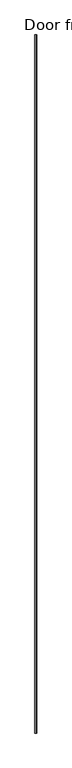
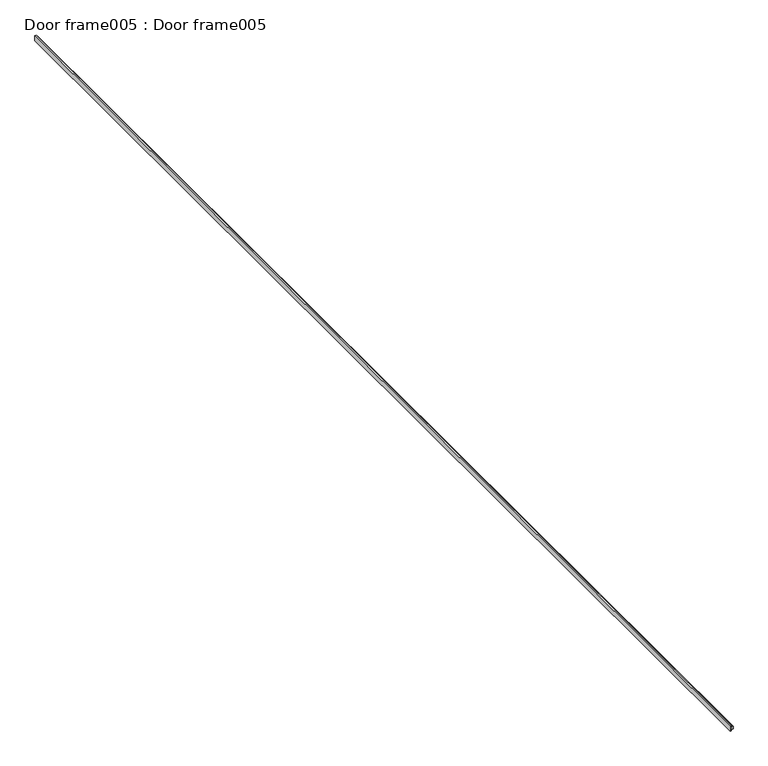
"""IFC4 building model written with IfcOpenShell, lengths in millimetres: proxy geometry, Door frame005 : Door frame005."""

import ifcopenshell
import ifcopenshell.guid

model = None  # the IFC model being written
_history = None  # IfcOwnerHistory: only IFC2X3 demands one
_inside = {}  # id of a spatial element -> (the spatial element, [elements in it])
_under = {}  # id of a project, library or spatial element -> (it, [spatial elements below it])
_declared = {}  # id of a project -> (the project, [libraries it declares])
_typed = {}  # id of a type object -> (the type object, [elements of that type])
_made_of = {}  # id of a material, layer set ... -> (it, [elements and type objects made of it])


def new_model(schema):
    """Start an empty IFC model of exactly this schema.

    Asked for "IFC4X3", IfcOpenShell would pick the latest addendum, in which some entities
    have other attributes; the version numbers below select the first issue.
    IFC2X3 requires an IfcOwnerHistory on every rooted entity: one is made here for all.
    """
    global model, _history
    if schema == "IFC4X3":
        model = ifcopenshell.file(schema_version=(4, 3, 0, 0))
    else:
        model = ifcopenshell.file(schema=schema)
    _inside.clear()
    _under.clear()
    _declared.clear()
    _typed.clear()
    _made_of.clear()
    _history = None
    if model.schema == "IFC2X3":
        org = make("IfcOrganization", Name="unknown")
        user = make(
            "IfcPersonAndOrganization",
            ThePerson=make("IfcPerson", FamilyName="unknown"),
            TheOrganization=org,
        )
        app = make(
            "IfcApplication",
            ApplicationDeveloper=org,
            Version="unknown",
            ApplicationFullName="unknown",
            ApplicationIdentifier="unknown",
        )
        _history = make(
            "IfcOwnerHistory",
            OwningUser=user,
            OwningApplication=app,
            ChangeAction="ADDED",
            CreationDate=0,
        )
    return model


def make(cls, **values):
    """One entity of the class cls with the attributes given. An attribute that is None is left unset."""
    return model.create_entity(
        cls, **{name: value for name, value in values.items() if value is not None}
    )


def rooted(cls, **values):
    """An entity with a GlobalId (a new one), such as an element, a storey or a relation."""
    return make(cls, GlobalId=ifcopenshell.guid.new(), OwnerHistory=_history, **values)


def si_unit(unit_type, name, prefix=None):
    """IfcSIUnit, for example si_unit("LENGTHUNIT", "METRE", prefix="MILLI")."""
    return make("IfcSIUnit", UnitType=unit_type, Prefix=prefix, Name=name)


def assignment(units):
    """IfcUnitAssignment: the units of a project."""
    return None if units is None else make("IfcUnitAssignment", Units=units)


def point(xyz):
    """IfcCartesianPoint."""
    return None if xyz is None else make("IfcCartesianPoint", Coordinates=xyz)


def direction(xyz):
    """IfcDirection."""
    return None if xyz is None else make("IfcDirection", DirectionRatios=xyz)


def frame(location, z_axis=None, x_axis=None):
    """IfcAxis2Placement3D, a coordinate frame: its origin and axes. An axis left out is left unset."""
    return make(
        "IfcAxis2Placement3D",
        Location=point(location),
        Axis=direction(z_axis),
        RefDirection=direction(x_axis),
    )


def origin():
    """The frame at (0, 0, 0) with its axes left unset."""
    return frame((0.0, 0.0, 0.0))


def place(relative_to, where):
    """IfcLocalPlacement: puts the frame where relative to a parent placement (None: the world)."""
    return make(
        "IfcLocalPlacement", PlacementRelTo=relative_to, RelativePlacement=where
    )


def context(
    kind, dimensions, precision=None, world=None, true_north=None, identifier=None
):
    """IfcGeometricRepresentationContext, for example the 3D "Model" context."""
    return make(
        "IfcGeometricRepresentationContext",
        ContextIdentifier=identifier,
        ContextType=kind,
        CoordinateSpaceDimension=dimensions,
        Precision=precision,
        WorldCoordinateSystem=world,
        TrueNorth=true_north,
    )


def project(units=None, contexts=None):
    """IfcProject with its units and contexts."""
    return rooted(
        "IfcProject",
        Name="project",
        RepresentationContexts=contexts,
        UnitsInContext=assignment(units),
    )


def spatial(cls, under=None, at=None, **own):
    """A site, building, storey or space (cls), placed at a placement, below another one or the project."""
    s = rooted(cls, ObjectPlacement=at, **own)
    if under is not None:
        _under.setdefault(under.id(), (under, []))[1].append(s)
    return s


def polyline(points):
    """IfcPolyline through the points."""
    return make("IfcPolyline", Points=[point(p) for p in points])


def outline(outer, holes=None, kind="AREA"):
    """IfcArbitraryClosedProfileDef: a profile drawn as a closed curve; with holes, ...WithVoids."""
    if holes is None:
        return make("IfcArbitraryClosedProfileDef", ProfileType=kind, OuterCurve=outer)
    return make(
        "IfcArbitraryProfileDefWithVoids",
        ProfileType=kind,
        OuterCurve=outer,
        InnerCurves=holes,
    )


def extrude(swept, where, along, depth):
    """IfcExtrudedAreaSolid: the profile swept, set in the frame where, extruded along a direction by depth."""
    return make(
        "IfcExtrudedAreaSolid",
        SweptArea=swept,
        Position=where,
        ExtrudedDirection=direction(along),
        Depth=depth,
    )


def shape(context_of_items, identifier, shape_type, items):
    """IfcShapeRepresentation: the items that make up one representation, for example the "Body"."""
    return make(
        "IfcShapeRepresentation",
        ContextOfItems=context_of_items,
        RepresentationIdentifier=identifier,
        RepresentationType=shape_type,
        Items=items,
    )


def source(mapping_origin, context_of_items, identifier, shape_type, items):
    """IfcRepresentationMap: a shape defined once, which mapped items show again and again."""
    return make(
        "IfcRepresentationMap",
        MappingOrigin=mapping_origin,
        MappedRepresentation=shape(context_of_items, identifier, shape_type, items),
    )


def transform(
    local_origin,
    x_axis=None,
    y_axis=None,
    z_axis=None,
    scale=None,
    scale2=None,
    scale3=None,
    uniform=True,
):
    """IfcCartesianTransformationOperator3D, or its non-uniform kind. x_axis, y_axis, z_axis: its Axis1, 2, 3."""
    if uniform:
        return make(
            "IfcCartesianTransformationOperator3D",
            Axis1=direction(x_axis),
            Axis2=direction(y_axis),
            LocalOrigin=point(local_origin),
            Scale=scale,
            Axis3=direction(z_axis),
        )
    return make(
        "IfcCartesianTransformationOperator3DnonUniform",
        Axis1=direction(x_axis),
        Axis2=direction(y_axis),
        LocalOrigin=point(local_origin),
        Scale=scale,
        Axis3=direction(z_axis),
        Scale2=scale2,
        Scale3=scale3,
    )


def mapped(mapping_source, mapping_target):
    """IfcMappedItem: shows the shape of a source again, moved by a transform."""
    return make(
        "IfcMappedItem", MappingSource=mapping_source, MappingTarget=mapping_target
    )


def made_of(thing, what):
    """Note that an element or type object is made of a material, layer set ...; save() writes the relation."""
    if what is not None:
        _made_of.setdefault(what.id(), (what, []))[1].append(thing)
    return thing


def element(
    cls,
    number,
    at=None,
    inside=None,
    cuts=None,
    type_object=None,
    material=None,
    context=None,
    identifier="Body",
    shape_type=None,
    held_by="IfcProductDefinitionShape",
    body=None,
    shapes=None,
    **own,
):
    """One element of the class cls, such as IfcWall. Its Tag is "e" and its number.

    at: its placement. inside: the storey or other place that contains it. cuts: it is an
    opening in that element (IfcRelVoidsElement). A single representation is given by context,
    identifier, shape_type and body (its items); several are given by shapes. held_by: the class
    of the entity that holds the representations. save() writes the other relations.
    """
    e = rooted(cls, Tag="e%d" % number, ObjectPlacement=at, **own)
    if body is not None:
        shapes = [shape(context, identifier, shape_type, body)]
    if shapes is not None:
        e.Representation = make(held_by, Representations=shapes)
    if inside is not None:
        _inside.setdefault(inside.id(), (inside, []))[1].append(e)
    if cuts is not None:
        rooted(
            "IfcRelVoidsElement", RelatingBuildingElement=cuts, RelatedOpeningElement=e
        )
    if type_object is not None:
        _typed.setdefault(type_object.id(), (type_object, []))[1].append(e)
    return made_of(e, material)


def aggregate(whole, parts):
    """IfcRelAggregates: a whole, such as a stair, and the parts it consists of."""
    return rooted("IfcRelAggregates", RelatingObject=whole, RelatedObjects=parts)


def save(model, path):
    """Write the relations noted so far, then the file.

    IfcRelAggregates (storeys below a building ...), IfcRelContainedInSpatialStructure (elements
    in a storey), IfcRelDefinesByType, IfcRelAssociatesMaterial and IfcRelDeclares: one each for
    every whole, place, type object, material and project.
    """
    for whole, parts in _under.values():
        aggregate(whole, parts)
    for where, things in _inside.values():
        rooted(
            "IfcRelContainedInSpatialStructure",
            RelatedElements=things,
            RelatingStructure=where,
        )
    for kind, things in _typed.values():
        rooted("IfcRelDefinesByType", RelatedObjects=things, RelatingType=kind)
    for what, things in _made_of.values():
        rooted("IfcRelAssociatesMaterial", RelatedObjects=things, RelatingMaterial=what)
    for by, libraries in _declared.values():
        rooted("IfcRelDeclares", RelatingContext=by, RelatedDefinitions=libraries)
    model.write(path)


def door_frame005_door_frame005_abb10e86(model_context):
    return source(origin(), model_context, "Body", "SweptSolid", [
        extrude(outline(polyline([(36678.7014343, 15555.3292246), (36678.7014343, 15557.5465976), (36682.2000947, 15557.5465976), (36682.2000947, 15559.3245976), (36680.8030947, 15559.3245976), (36680.8030947, 15560.3913976), (36685.3750947, 15560.3913976), (36685.3750947, 15559.3245976), (36683.9780947, 15559.3245976), (36683.9780947, 15557.546547), (36687.4772673, 15557.546547), (36687.4772673, 15555.3292246), (36678.7014343, 15555.3292246)])), frame((0.0, -1052.8906567, 0.0), z_axis=(0.0, 1.0, 0.0), x_axis=(0.0, 0.0, 1.0)), (0.0, 0.0, 1.0), 1999.85),
    ])


if __name__ == "__main__":
    model = new_model("IFC4")
    model_context = context("Model", 3, world=origin())
    ifc_project = project(units=[si_unit("LENGTHUNIT", "METRE", prefix="MILLI")], contexts=[model_context])
    site = spatial("IfcSite", under=ifc_project)
    building = spatial("IfcBuilding", under=site)
    placement = place(None, origin())
    door_frame005_door_frame005_shape = door_frame005_door_frame005_abb10e86(model_context)
    element("IfcBuildingElementProxy", 1, Name="Door frame005 : Door frame005", ObjectType="Door frame005 : Door frame005", at=placement, inside=building, context=model_context, shape_type="MappedRepresentation", body=[
        mapped(door_frame005_door_frame005_shape, transform((0.0, 0.0, 0.0), x_axis=(1.0, 0.0, 0.0), y_axis=(0.0, 1.0, 0.0), z_axis=(0.0, 0.0, 1.0))),
    ])
    save(model, "model.ifc")

# Revit data of these elements
# Type "Door frame005 : Door frame005"
#   NameOverride = "Door frame005"
# Element 1 (IfcBuildingElementProxy, "Door frame005 : Door frame005")
#   Materials on its faces: "FLEETWOOD SERIES T-3200 SINGLE SWING DOOR FRAME"
# Materials
#   "FLEETWOOD SERIES T-3200 SINGLE SWING DOOR FRAME": class "Unassigned", colour RGB 128 128 128, transparency 0, Cost = 0
